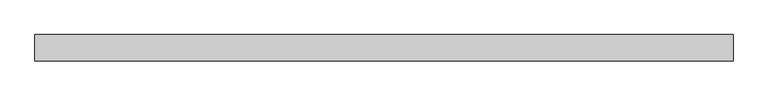
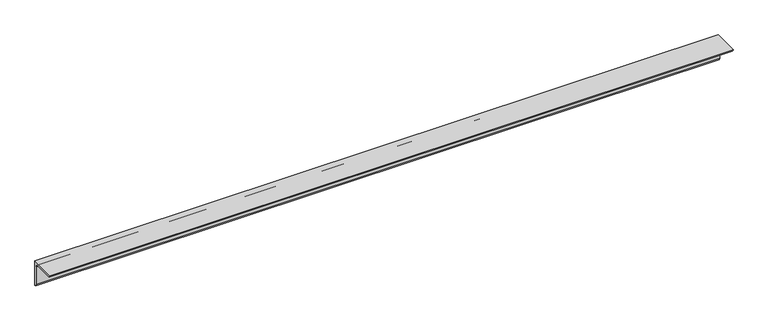
"""IFC4 building model written with IfcOpenShell, lengths in millimetres: member geometry, 0912_Steel Framing_L-KSD3502 : H_SB_AR_S03_L-130x130x12_HBR3."""

import ifcopenshell
import ifcopenshell.guid

model = None  # the IFC model being written
_history = None  # IfcOwnerHistory: only IFC2X3 demands one
_inside = {}  # id of a spatial element -> (the spatial element, [elements in it])
_under = {}  # id of a project, library or spatial element -> (it, [spatial elements below it])
_declared = {}  # id of a project -> (the project, [libraries it declares])
_typed = {}  # id of a type object -> (the type object, [elements of that type])
_made_of = {}  # id of a material, layer set ... -> (it, [elements and type objects made of it])


def new_model(schema):
    """Start an empty IFC model of exactly this schema.

    Asked for "IFC4X3", IfcOpenShell would pick the latest addendum, in which some entities
    have other attributes; the version numbers below select the first issue.
    IFC2X3 requires an IfcOwnerHistory on every rooted entity: one is made here for all.
    """
    global model, _history
    if schema == "IFC4X3":
        model = ifcopenshell.file(schema_version=(4, 3, 0, 0))
    else:
        model = ifcopenshell.file(schema=schema)
    _inside.clear()
    _under.clear()
    _declared.clear()
    _typed.clear()
    _made_of.clear()
    _history = None
    if model.schema == "IFC2X3":
        org = make("IfcOrganization", Name="unknown")
        user = make(
            "IfcPersonAndOrganization",
            ThePerson=make("IfcPerson", FamilyName="unknown"),
            TheOrganization=org,
        )
        app = make(
            "IfcApplication",
            ApplicationDeveloper=org,
            Version="unknown",
            ApplicationFullName="unknown",
            ApplicationIdentifier="unknown",
        )
        _history = make(
            "IfcOwnerHistory",
            OwningUser=user,
            OwningApplication=app,
            ChangeAction="ADDED",
            CreationDate=0,
        )
    return model


def make(cls, **values):
    """One entity of the class cls with the attributes given. An attribute that is None is left unset."""
    return model.create_entity(
        cls, **{name: value for name, value in values.items() if value is not None}
    )


def rooted(cls, **values):
    """An entity with a GlobalId (a new one), such as an element, a storey or a relation."""
    return make(cls, GlobalId=ifcopenshell.guid.new(), OwnerHistory=_history, **values)


def si_unit(unit_type, name, prefix=None):
    """IfcSIUnit, for example si_unit("LENGTHUNIT", "METRE", prefix="MILLI")."""
    return make("IfcSIUnit", UnitType=unit_type, Prefix=prefix, Name=name)


def assignment(units):
    """IfcUnitAssignment: the units of a project."""
    return None if units is None else make("IfcUnitAssignment", Units=units)


def point(xyz):
    """IfcCartesianPoint."""
    return None if xyz is None else make("IfcCartesianPoint", Coordinates=xyz)


def direction(xyz):
    """IfcDirection."""
    return None if xyz is None else make("IfcDirection", DirectionRatios=xyz)


def frame(location, z_axis=None, x_axis=None):
    """IfcAxis2Placement3D, a coordinate frame: its origin and axes. An axis left out is left unset."""
    return make(
        "IfcAxis2Placement3D",
        Location=point(location),
        Axis=direction(z_axis),
        RefDirection=direction(x_axis),
    )


def frame_2d(location, x_axis=None):
    """IfcAxis2Placement2D, a coordinate frame in the plane: its origin and x axis."""
    return make(
        "IfcAxis2Placement2D", Location=point(location), RefDirection=direction(x_axis)
    )


def origin():
    """The frame at (0, 0, 0) with its axes left unset."""
    return frame((0.0, 0.0, 0.0))


def place(relative_to, where):
    """IfcLocalPlacement: puts the frame where relative to a parent placement (None: the world)."""
    return make(
        "IfcLocalPlacement", PlacementRelTo=relative_to, RelativePlacement=where
    )


def context(
    kind, dimensions, precision=None, world=None, true_north=None, identifier=None
):
    """IfcGeometricRepresentationContext, for example the 3D "Model" context."""
    return make(
        "IfcGeometricRepresentationContext",
        ContextIdentifier=identifier,
        ContextType=kind,
        CoordinateSpaceDimension=dimensions,
        Precision=precision,
        WorldCoordinateSystem=world,
        TrueNorth=true_north,
    )


def project(units=None, contexts=None):
    """IfcProject with its units and contexts."""
    return rooted(
        "IfcProject",
        Name="project",
        RepresentationContexts=contexts,
        UnitsInContext=assignment(units),
    )


def spatial(cls, under=None, at=None, **own):
    """A site, building, storey or space (cls), placed at a placement, below another one or the project."""
    s = rooted(cls, ObjectPlacement=at, **own)
    if under is not None:
        _under.setdefault(under.id(), (under, []))[1].append(s)
    return s


def polyline(points):
    """IfcPolyline through the points."""
    return make("IfcPolyline", Points=[point(p) for p in points])


def circle_curve(where, radius):
    """IfcCircle in the frame where."""
    return make("IfcCircle", Position=where, Radius=radius)


def trimmed(basis, trim1, trim2, sense, master):
    """IfcTrimmedCurve: the piece of a basis curve between two trims."""
    return make(
        "IfcTrimmedCurve",
        BasisCurve=basis,
        Trim1=trim1,
        Trim2=trim2,
        SenseAgreement=sense,
        MasterRepresentation=master,
    )


def segment(curve, same_sense, transition):
    """IfcCompositeCurveSegment."""
    return make(
        "IfcCompositeCurveSegment",
        Transition=transition,
        SameSense=same_sense,
        ParentCurve=curve,
    )


def composite_curve(segments, self_intersect=None):
    """IfcCompositeCurve: segments joined end to end."""
    return make("IfcCompositeCurve", Segments=segments, SelfIntersect=self_intersect)


def outline(outer, holes=None, kind="AREA"):
    """IfcArbitraryClosedProfileDef: a profile drawn as a closed curve; with holes, ...WithVoids."""
    if holes is None:
        return make("IfcArbitraryClosedProfileDef", ProfileType=kind, OuterCurve=outer)
    return make(
        "IfcArbitraryProfileDefWithVoids",
        ProfileType=kind,
        OuterCurve=outer,
        InnerCurves=holes,
    )


def extrude(swept, where, along, depth):
    """IfcExtrudedAreaSolid: the profile swept, set in the frame where, extruded along a direction by depth."""
    return make(
        "IfcExtrudedAreaSolid",
        SweptArea=swept,
        Position=where,
        ExtrudedDirection=direction(along),
        Depth=depth,
    )


def shape(context_of_items, identifier, shape_type, items):
    """IfcShapeRepresentation: the items that make up one representation, for example the "Body"."""
    return make(
        "IfcShapeRepresentation",
        ContextOfItems=context_of_items,
        RepresentationIdentifier=identifier,
        RepresentationType=shape_type,
        Items=items,
    )


def source(mapping_origin, context_of_items, identifier, shape_type, items):
    """IfcRepresentationMap: a shape defined once, which mapped items show again and again."""
    return make(
        "IfcRepresentationMap",
        MappingOrigin=mapping_origin,
        MappedRepresentation=shape(context_of_items, identifier, shape_type, items),
    )


def transform(
    local_origin,
    x_axis=None,
    y_axis=None,
    z_axis=None,
    scale=None,
    scale2=None,
    scale3=None,
    uniform=True,
):
    """IfcCartesianTransformationOperator3D, or its non-uniform kind. x_axis, y_axis, z_axis: its Axis1, 2, 3."""
    if uniform:
        return make(
            "IfcCartesianTransformationOperator3D",
            Axis1=direction(x_axis),
            Axis2=direction(y_axis),
            LocalOrigin=point(local_origin),
            Scale=scale,
            Axis3=direction(z_axis),
        )
    return make(
        "IfcCartesianTransformationOperator3DnonUniform",
        Axis1=direction(x_axis),
        Axis2=direction(y_axis),
        LocalOrigin=point(local_origin),
        Scale=scale,
        Axis3=direction(z_axis),
        Scale2=scale2,
        Scale3=scale3,
    )


def mapped(mapping_source, mapping_target):
    """IfcMappedItem: shows the shape of a source again, moved by a transform."""
    return make(
        "IfcMappedItem", MappingSource=mapping_source, MappingTarget=mapping_target
    )


def made_of(thing, what):
    """Note that an element or type object is made of a material, layer set ...; save() writes the relation."""
    if what is not None:
        _made_of.setdefault(what.id(), (what, []))[1].append(thing)
    return thing


def element(
    cls,
    number,
    at=None,
    inside=None,
    cuts=None,
    type_object=None,
    material=None,
    context=None,
    identifier="Body",
    shape_type=None,
    held_by="IfcProductDefinitionShape",
    body=None,
    shapes=None,
    **own,
):
    """One element of the class cls, such as IfcWall. Its Tag is "e" and its number.

    at: its placement. inside: the storey or other place that contains it. cuts: it is an
    opening in that element (IfcRelVoidsElement). A single representation is given by context,
    identifier, shape_type and body (its items); several are given by shapes. held_by: the class
    of the entity that holds the representations. save() writes the other relations.
    """
    e = rooted(cls, Tag="e%d" % number, ObjectPlacement=at, **own)
    if body is not None:
        shapes = [shape(context, identifier, shape_type, body)]
    if shapes is not None:
        e.Representation = make(held_by, Representations=shapes)
    if inside is not None:
        _inside.setdefault(inside.id(), (inside, []))[1].append(e)
    if cuts is not None:
        rooted(
            "IfcRelVoidsElement", RelatingBuildingElement=cuts, RelatedOpeningElement=e
        )
    if type_object is not None:
        _typed.setdefault(type_object.id(), (type_object, []))[1].append(e)
    return made_of(e, material)


def aggregate(whole, parts):
    """IfcRelAggregates: a whole, such as a stair, and the parts it consists of."""
    return rooted("IfcRelAggregates", RelatingObject=whole, RelatedObjects=parts)


def save(model, path):
    """Write the relations noted so far, then the file.

    IfcRelAggregates (storeys below a building ...), IfcRelContainedInSpatialStructure (elements
    in a storey), IfcRelDefinesByType, IfcRelAssociatesMaterial and IfcRelDeclares: one each for
    every whole, place, type object, material and project.
    """
    for whole, parts in _under.values():
        aggregate(whole, parts)
    for where, things in _inside.values():
        rooted(
            "IfcRelContainedInSpatialStructure",
            RelatedElements=things,
            RelatingStructure=where,
        )
    for kind, things in _typed.values():
        rooted("IfcRelDefinesByType", RelatedObjects=things, RelatingType=kind)
    for what, things in _made_of.values():
        rooted("IfcRelAssociatesMaterial", RelatedObjects=things, RelatingMaterial=what)
    for by, libraries in _declared.values():
        rooted("IfcRelDeclares", RelatingContext=by, RelatedDefinitions=libraries)
    model.write(path)


def member_336a097f(model_context):
    return source(origin(), model_context, "Body", "SweptSolid", [
        extrude(outline(composite_curve([segment(polyline([(36.4, 36.4), (36.4, -93.6)]), True, "CONTINUOUS"), segment(trimmed(circle_curve(frame_2d((36.4, -81.6)), 12.0), [point((36.4, -93.6))], [point((24.4, -81.6))], False, "CARTESIAN"), True, "CONTINUOUS"), segment(polyline([(24.4, -81.6), (24.4, 12.4)]), True, "CONTINUOUS"), segment(trimmed(circle_curve(frame_2d((12.4, 12.4)), 12.0), [point((24.4, 12.4))], [point((12.4, 24.4))], True, "CARTESIAN"), True, "CONTINUOUS"), segment(polyline([(12.4, 24.4), (-81.6, 24.4)]), True, "CONTINUOUS"), segment(trimmed(circle_curve(frame_2d((-81.6, 36.4)), 12.0), [point((-81.6, 24.4))], [point((-93.6, 36.4))], False, "CARTESIAN"), True, "CONTINUOUS"), segment(polyline([(-93.6, 36.4), (36.4, 36.4)]), True, "CONTINUOUS")], self_intersect=False)), frame((-1734.7763172, 0.0, 0.0), z_axis=(1.0, 0.0, 0.0), x_axis=(0.0, 1.0, 0.0)), (0.0, 0.0, 1.0), 3433.9208324),
    ])


if __name__ == "__main__":
    model = new_model("IFC4")
    model_context = context("Model", 3, world=origin())
    ifc_project = project(units=[si_unit("LENGTHUNIT", "METRE", prefix="MILLI")], contexts=[model_context])
    site = spatial("IfcSite", under=ifc_project)
    building = spatial("IfcBuilding", under=site)
    placement = place(None, origin())
    member_shape = member_336a097f(model_context)
    element("IfcMember", 1, ObjectType="0912_Steel Framing_L-KSD3502 : H_SB_AR_S03_L-130x130x12_HBR3", at=placement, inside=building, context=model_context, shape_type="MappedRepresentation", body=[
        mapped(member_shape, transform((0.0, 0.0, 0.0), x_axis=(1.0, 0.0, 0.0), y_axis=(0.0, 1.0, 0.0), z_axis=(0.0, 0.0, 1.0))),
    ])
    save(model, "model.ifc")

# Revit data of these elements
# Type "0912_Steel Framing_L-KSD3502 : H_SB_AR_S03_L-130x130x12_HBR3"
#   k = 25 mm
#   Perimeter = 0.52 m²/m
#   Nominal Weight = 23.40 kgf/m
#   Length [instance default] = 1000 mm
#   b = 130 mm
#   d = 130 mm
#   t = 12 mm
#   x = 36.4 mm
#   y = 36.4 mm
#   A = 2976.00 m²
#   Structural Material [instance default] = Steel, 45-345
# Element 1 (IfcMember, "0912_Steel Framing_L-KSD3502 : H_SB_AR_S03_L-130x130x12_HBR3")
#   Structural Material = Steel ASTM A36
#   Materials on its faces: "Steel ASTM A36"
# Materials
#   "Steel, 45-345": class "Metal", colour RGB 189 187 185, transparency 0, Description = "Steel 345 MPa", Cost = 0
#   "Steel ASTM A36": class "Metal", colour RGB 199 199 199, transparency 0, Description = "Structural steel, ASTM A36 Grade B, mill finish", Cost = 0
